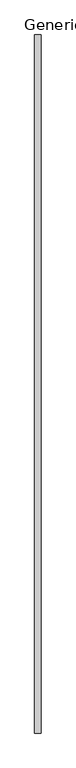
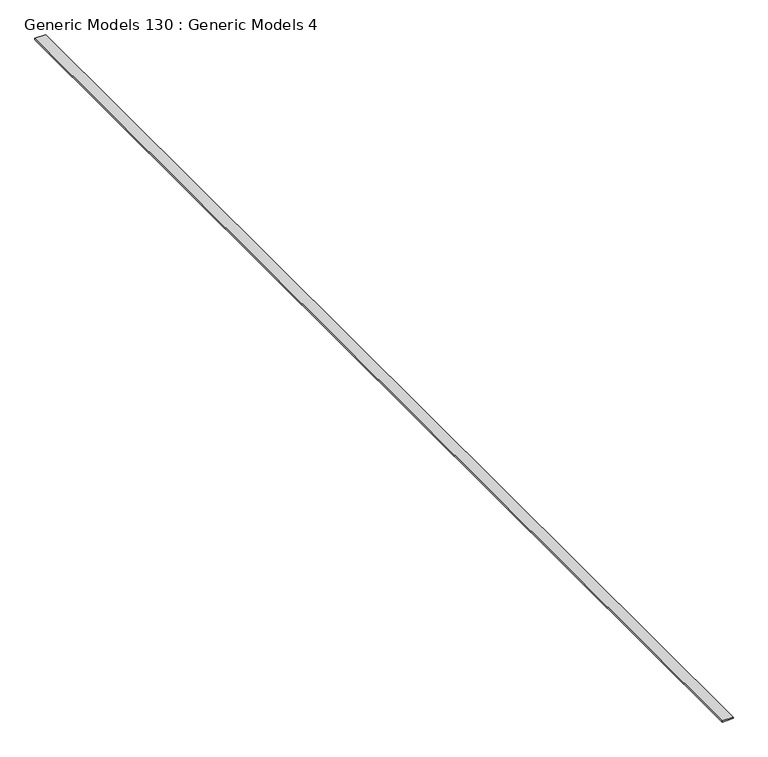
"""IFC4 building model written with IfcOpenShell, lengths in millimetres: proxy geometry, Generic Models 130 : Generic Models 4."""

import ifcopenshell
import ifcopenshell.guid

model = None  # the IFC model being written
_history = None  # IfcOwnerHistory: only IFC2X3 demands one
_inside = {}  # id of a spatial element -> (the spatial element, [elements in it])
_under = {}  # id of a project, library or spatial element -> (it, [spatial elements below it])
_declared = {}  # id of a project -> (the project, [libraries it declares])
_typed = {}  # id of a type object -> (the type object, [elements of that type])
_made_of = {}  # id of a material, layer set ... -> (it, [elements and type objects made of it])


def new_model(schema):
    """Start an empty IFC model of exactly this schema.

    Asked for "IFC4X3", IfcOpenShell would pick the latest addendum, in which some entities
    have other attributes; the version numbers below select the first issue.
    IFC2X3 requires an IfcOwnerHistory on every rooted entity: one is made here for all.
    """
    global model, _history
    if schema == "IFC4X3":
        model = ifcopenshell.file(schema_version=(4, 3, 0, 0))
    else:
        model = ifcopenshell.file(schema=schema)
    _inside.clear()
    _under.clear()
    _declared.clear()
    _typed.clear()
    _made_of.clear()
    _history = None
    if model.schema == "IFC2X3":
        org = make("IfcOrganization", Name="unknown")
        user = make(
            "IfcPersonAndOrganization",
            ThePerson=make("IfcPerson", FamilyName="unknown"),
            TheOrganization=org,
        )
        app = make(
            "IfcApplication",
            ApplicationDeveloper=org,
            Version="unknown",
            ApplicationFullName="unknown",
            ApplicationIdentifier="unknown",
        )
        _history = make(
            "IfcOwnerHistory",
            OwningUser=user,
            OwningApplication=app,
            ChangeAction="ADDED",
            CreationDate=0,
        )
    return model


def make(cls, **values):
    """One entity of the class cls with the attributes given. An attribute that is None is left unset."""
    return model.create_entity(
        cls, **{name: value for name, value in values.items() if value is not None}
    )


def rooted(cls, **values):
    """An entity with a GlobalId (a new one), such as an element, a storey or a relation."""
    return make(cls, GlobalId=ifcopenshell.guid.new(), OwnerHistory=_history, **values)


def si_unit(unit_type, name, prefix=None):
    """IfcSIUnit, for example si_unit("LENGTHUNIT", "METRE", prefix="MILLI")."""
    return make("IfcSIUnit", UnitType=unit_type, Prefix=prefix, Name=name)


def assignment(units):
    """IfcUnitAssignment: the units of a project."""
    return None if units is None else make("IfcUnitAssignment", Units=units)


def point(xyz):
    """IfcCartesianPoint."""
    return None if xyz is None else make("IfcCartesianPoint", Coordinates=xyz)


def direction(xyz):
    """IfcDirection."""
    return None if xyz is None else make("IfcDirection", DirectionRatios=xyz)


def frame(location, z_axis=None, x_axis=None):
    """IfcAxis2Placement3D, a coordinate frame: its origin and axes. An axis left out is left unset."""
    return make(
        "IfcAxis2Placement3D",
        Location=point(location),
        Axis=direction(z_axis),
        RefDirection=direction(x_axis),
    )


def origin():
    """The frame at (0, 0, 0) with its axes left unset."""
    return frame((0.0, 0.0, 0.0))


def place(relative_to, where):
    """IfcLocalPlacement: puts the frame where relative to a parent placement (None: the world)."""
    return make(
        "IfcLocalPlacement", PlacementRelTo=relative_to, RelativePlacement=where
    )


def context(
    kind, dimensions, precision=None, world=None, true_north=None, identifier=None
):
    """IfcGeometricRepresentationContext, for example the 3D "Model" context."""
    return make(
        "IfcGeometricRepresentationContext",
        ContextIdentifier=identifier,
        ContextType=kind,
        CoordinateSpaceDimension=dimensions,
        Precision=precision,
        WorldCoordinateSystem=world,
        TrueNorth=true_north,
    )


def project(units=None, contexts=None):
    """IfcProject with its units and contexts."""
    return rooted(
        "IfcProject",
        Name="project",
        RepresentationContexts=contexts,
        UnitsInContext=assignment(units),
    )


def spatial(cls, under=None, at=None, **own):
    """A site, building, storey or space (cls), placed at a placement, below another one or the project."""
    s = rooted(cls, ObjectPlacement=at, **own)
    if under is not None:
        _under.setdefault(under.id(), (under, []))[1].append(s)
    return s


def polyline(points):
    """IfcPolyline through the points."""
    return make("IfcPolyline", Points=[point(p) for p in points])


def outline(outer, holes=None, kind="AREA"):
    """IfcArbitraryClosedProfileDef: a profile drawn as a closed curve; with holes, ...WithVoids."""
    if holes is None:
        return make("IfcArbitraryClosedProfileDef", ProfileType=kind, OuterCurve=outer)
    return make(
        "IfcArbitraryProfileDefWithVoids",
        ProfileType=kind,
        OuterCurve=outer,
        InnerCurves=holes,
    )


def extrude(swept, where, along, depth):
    """IfcExtrudedAreaSolid: the profile swept, set in the frame where, extruded along a direction by depth."""
    return make(
        "IfcExtrudedAreaSolid",
        SweptArea=swept,
        Position=where,
        ExtrudedDirection=direction(along),
        Depth=depth,
    )


def shape(context_of_items, identifier, shape_type, items):
    """IfcShapeRepresentation: the items that make up one representation, for example the "Body"."""
    return make(
        "IfcShapeRepresentation",
        ContextOfItems=context_of_items,
        RepresentationIdentifier=identifier,
        RepresentationType=shape_type,
        Items=items,
    )


def source(mapping_origin, context_of_items, identifier, shape_type, items):
    """IfcRepresentationMap: a shape defined once, which mapped items show again and again."""
    return make(
        "IfcRepresentationMap",
        MappingOrigin=mapping_origin,
        MappedRepresentation=shape(context_of_items, identifier, shape_type, items),
    )


def transform(
    local_origin,
    x_axis=None,
    y_axis=None,
    z_axis=None,
    scale=None,
    scale2=None,
    scale3=None,
    uniform=True,
):
    """IfcCartesianTransformationOperator3D, or its non-uniform kind. x_axis, y_axis, z_axis: its Axis1, 2, 3."""
    if uniform:
        return make(
            "IfcCartesianTransformationOperator3D",
            Axis1=direction(x_axis),
            Axis2=direction(y_axis),
            LocalOrigin=point(local_origin),
            Scale=scale,
            Axis3=direction(z_axis),
        )
    return make(
        "IfcCartesianTransformationOperator3DnonUniform",
        Axis1=direction(x_axis),
        Axis2=direction(y_axis),
        LocalOrigin=point(local_origin),
        Scale=scale,
        Axis3=direction(z_axis),
        Scale2=scale2,
        Scale3=scale3,
    )


def mapped(mapping_source, mapping_target):
    """IfcMappedItem: shows the shape of a source again, moved by a transform."""
    return make(
        "IfcMappedItem", MappingSource=mapping_source, MappingTarget=mapping_target
    )


def made_of(thing, what):
    """Note that an element or type object is made of a material, layer set ...; save() writes the relation."""
    if what is not None:
        _made_of.setdefault(what.id(), (what, []))[1].append(thing)
    return thing


def element(
    cls,
    number,
    at=None,
    inside=None,
    cuts=None,
    type_object=None,
    material=None,
    context=None,
    identifier="Body",
    shape_type=None,
    held_by="IfcProductDefinitionShape",
    body=None,
    shapes=None,
    **own,
):
    """One element of the class cls, such as IfcWall. Its Tag is "e" and its number.

    at: its placement. inside: the storey or other place that contains it. cuts: it is an
    opening in that element (IfcRelVoidsElement). A single representation is given by context,
    identifier, shape_type and body (its items); several are given by shapes. held_by: the class
    of the entity that holds the representations. save() writes the other relations.
    """
    e = rooted(cls, Tag="e%d" % number, ObjectPlacement=at, **own)
    if body is not None:
        shapes = [shape(context, identifier, shape_type, body)]
    if shapes is not None:
        e.Representation = make(held_by, Representations=shapes)
    if inside is not None:
        _inside.setdefault(inside.id(), (inside, []))[1].append(e)
    if cuts is not None:
        rooted(
            "IfcRelVoidsElement", RelatingBuildingElement=cuts, RelatedOpeningElement=e
        )
    if type_object is not None:
        _typed.setdefault(type_object.id(), (type_object, []))[1].append(e)
    return made_of(e, material)


def aggregate(whole, parts):
    """IfcRelAggregates: a whole, such as a stair, and the parts it consists of."""
    return rooted("IfcRelAggregates", RelatingObject=whole, RelatedObjects=parts)


def save(model, path):
    """Write the relations noted so far, then the file.

    IfcRelAggregates (storeys below a building ...), IfcRelContainedInSpatialStructure (elements
    in a storey), IfcRelDefinesByType, IfcRelAssociatesMaterial and IfcRelDeclares: one each for
    every whole, place, type object, material and project.
    """
    for whole, parts in _under.values():
        aggregate(whole, parts)
    for where, things in _inside.values():
        rooted(
            "IfcRelContainedInSpatialStructure",
            RelatedElements=things,
            RelatingStructure=where,
        )
    for kind, things in _typed.values():
        rooted("IfcRelDefinesByType", RelatedObjects=things, RelatingType=kind)
    for what, things in _made_of.values():
        rooted("IfcRelAssociatesMaterial", RelatedObjects=things, RelatingMaterial=what)
    for by, libraries in _declared.values():
        rooted("IfcRelDeclares", RelatingContext=by, RelatedDefinitions=libraries)
    model.write(path)


def generic_models_130_generic_models_4_d2a2c555(model_context):
    return source(origin(), model_context, "Body", "SweptSolid", [
        extrude(outline(polyline([(7338.4467872, -6864.9230338), (7169.2480051, -6864.9230338), (7169.2480051, 11778.6769662), (7338.4467872, 11778.6769662), (7338.4467872, -6864.9230338)])), frame((0.0, 0.0, 126524.8520404), z_axis=(0.0, 0.0, 1.0), x_axis=(1.0, 0.0, 0.0)), (0.0, 0.0, 1.0), 19.05),
    ])


if __name__ == "__main__":
    model = new_model("IFC4")
    model_context = context("Model", 3, world=origin())
    ifc_project = project(units=[si_unit("LENGTHUNIT", "METRE", prefix="MILLI")], contexts=[model_context])
    site = spatial("IfcSite", under=ifc_project)
    building = spatial("IfcBuilding", under=site)
    placement = place(None, origin())
    generic_models_130_generic_models_4_shape = generic_models_130_generic_models_4_d2a2c555(model_context)
    element("IfcBuildingElementProxy", 1, Name="Generic Models 130 : Generic Models 4", ObjectType="Generic Models 130 : Generic Models 4", at=placement, inside=building, context=model_context, shape_type="MappedRepresentation", body=[
        mapped(generic_models_130_generic_models_4_shape, transform((0.0, 0.0, 0.0), x_axis=(1.0, 0.0, 0.0), y_axis=(0.0, 1.0, 0.0), z_axis=(0.0, 0.0, 1.0))),
    ])
    save(model, "model.ifc")

# Revit data of these elements
# Element 1 (IfcBuildingElementProxy, "Generic Models 130 : Generic Models 4")
#   Materials on its faces: "_CDX PLYWOOD - SEE STRUCT DWGs"
# Materials
#   "_CDX PLYWOOD - SEE STRUCT DWGs": class "Generic", colour RGB 98 75 74, transparency 0, Cost = 0
